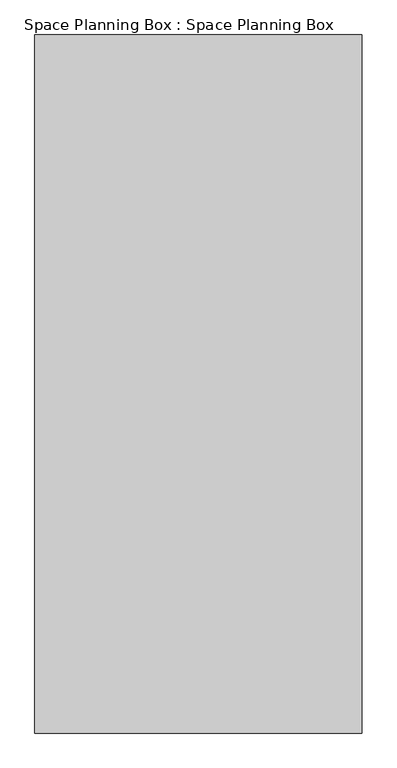
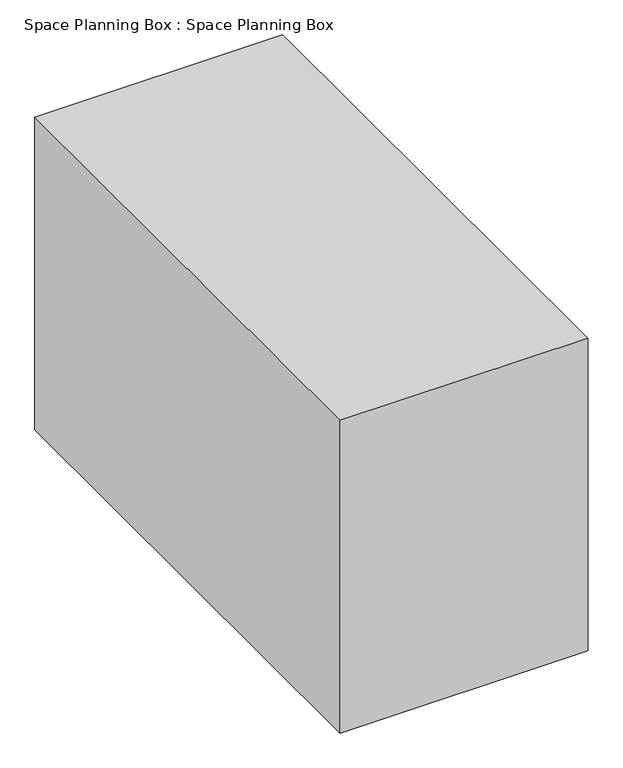
"""IFC4 building model written with IfcOpenShell, lengths in millimetres: proxy geometry, Space Planning Box : Space Planning Box."""

from ifc_helpers import new_model, si_unit, origin, origin_with_axes, place, context, project, spatial, polyline, outline, extrude, source, transform, mapped, element, save


def space_planning_box_space_planning_box_96097b63(model_context):
    return source(origin(), model_context, "Body", "SweptSolid", [
        extrude(outline(polyline([(2250.0, 4800.0), (2250.0, -4800.0), (-2250.0, -4800.0), (-2250.0, 4800.0), (2250.0, 4800.0)])), origin_with_axes(), (0.0, 0.0, 1.0), 6000.0),
    ])


if __name__ == "__main__":
    model = new_model("IFC4")
    model_context = context("Model", 3, world=origin())
    ifc_project = project(units=[si_unit("LENGTHUNIT", "METRE", prefix="MILLI")], contexts=[model_context])
    site = spatial("IfcSite", under=ifc_project)
    building = spatial("IfcBuilding", under=site)
    placement = place(None, origin())
    space_planning_box_space_planning_box_shape = space_planning_box_space_planning_box_96097b63(model_context)
    element("IfcBuildingElementProxy", 1, Name="Space Planning Box : Space Planning Box", ObjectType="Space Planning Box : Space Planning Box", at=placement, inside=building, context=model_context, shape_type="MappedRepresentation", body=[
        mapped(space_planning_box_space_planning_box_shape, transform((0.0, 0.0, 0.0), x_axis=(1.0, 0.0, 0.0), y_axis=(0.0, 1.0, 0.0), z_axis=(0.0, 0.0, 1.0))),
    ])
    save(model, "model.ifc")

# Revit data of these elements
# Type "Space Planning Box : Space Planning Box"
#   Type Comments = "..."
#   Room Name [instance default] = "?"
#   Assembly Code = "..."
#   Width [instance default] = 1524 mm
#   Program Area [instance default] = 0 m²
#   Length [instance default] = 1524 mm
#   Height [instance default] = 1524 mm
#   Area [instance default] = 2.32258 m²
#   Fill Color [instance default] = Cyan
#   Default Elevation = 0
# Element 1 (IfcBuildingElementProxy, "Space Planning Box : Space Planning Box")
#   Room Name = "Shift Office Room"
#   Width = 4500 mm
#   Program Area = 43.2 m²
#   Length = 9600 mm
#   Height = 6000 mm
#   Area = 43.2 m²
#   Fill Color = Lavender
#   Materials on its faces: "Lavender"
# Materials
#   "Cyan": class "Generic", colour RGB 0 255 255, transparency 0.2, Cost = 0
#   "Lavender": class "Generic", colour RGB 186 85 211, transparency 0.2, Cost = 0
